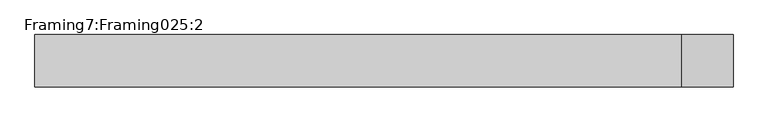
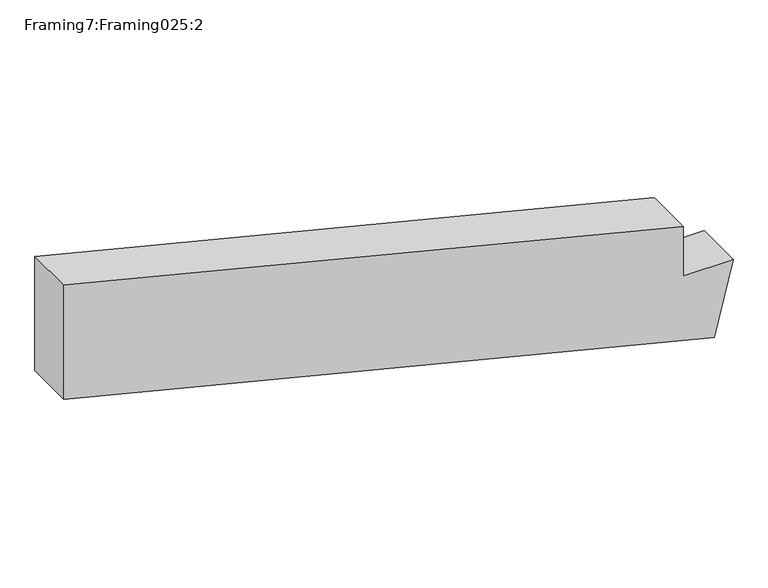
"""IFC4 building model written with IfcOpenShell, lengths in millimetres: proxy geometry, Framing7:Framing025:2 : Framing7:Framing025:286338."""

from ifc_helpers import new_model, si_unit, frame, origin, place, context, project, spatial, polyline, outline, extrude, source, transform, mapped, element, save


def framing7_framing025_2_fc919f43(model_context):
    return source(origin(), model_context, "Body", "SweptSolid", [
        extrude(outline(polyline([(110357.3362587, 15130.8894286), (110588.0006385, 15187.4083443), (110588.0006385, 15036.8413595), (110746.7842581, 15036.8413595), (111216.6873042, 13157.0903708), (110849.8516785, 13157.0903708), (110357.3362587, 15130.8894286)])), frame((0.0, -14445.349577, 0.0), z_axis=(0.0, 1.0, 0.0), x_axis=(0.0, 0.0, 1.0)), (0.0, 0.0, 1.0), 152.4),
    ])


if __name__ == "__main__":
    model = new_model("IFC4")
    model_context = context("Model", 3, world=origin())
    ifc_project = project(units=[si_unit("LENGTHUNIT", "METRE", prefix="MILLI")], contexts=[model_context])
    site = spatial("IfcSite", under=ifc_project)
    building = spatial("IfcBuilding", under=site)
    placement = place(None, origin())
    framing7_framing025_2_shape = framing7_framing025_2_fc919f43(model_context)
    element("IfcBuildingElementProxy", 1, Name="Framing7:Framing025:2 : Framing7:Framing025:286338", ObjectType="Framing7:Framing025:2 : Framing7:Framing025:286338", at=placement, inside=building, context=model_context, shape_type="MappedRepresentation", body=[
        mapped(framing7_framing025_2_shape, transform((0.0, 0.0, 0.0), x_axis=(1.0, 0.0, 0.0), y_axis=(0.0, 1.0, 0.0), z_axis=(0.0, 0.0, 1.0))),
    ])
    save(model, "model.ifc")

# Revit data of these elements
# Type "Framing7:Framing025:2 : Framing7:Framing025:286338"
#   NameOverride = "Framing7:Framing025:286338"
#   ObjectTypeOverride = "Framing7:Framing025"
#   Reference = "Framing025"
#   Category = "Generic Models"
#   Tag = "286338"
# Element 1 (IfcBuildingElementProxy, "Framing7:Framing025:2 : Framing7:Framing025:286338")
#   Materials on its faces: "WOOD FRAMING (SEE STRUCT DWGS)"
# Materials
#   "WOOD FRAMING (SEE STRUCT DWGS)": class "Unassigned", colour RGB 224 188 168, transparency 0, Cost = 0
